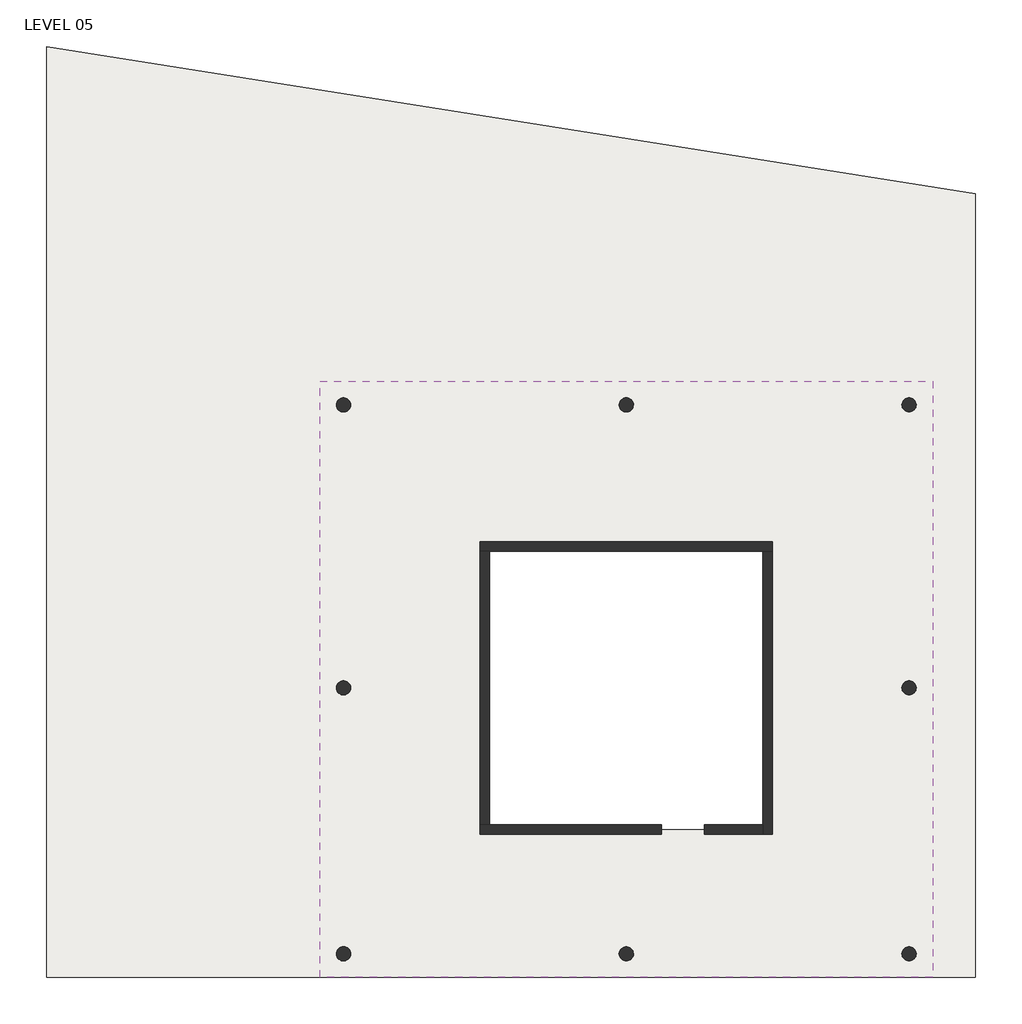
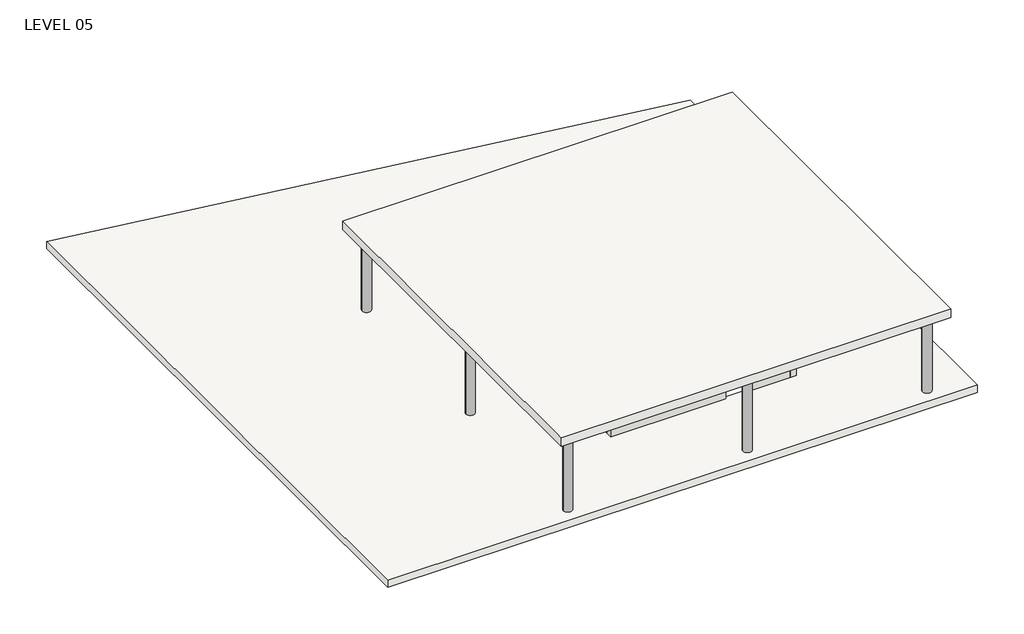
# One storey: 8 columns, 4 beams, 4 walls, 2 slabs.
"""IFC4 building model written with IfcOpenShell, lengths in millimetres."""

from ifc_helpers import new_model, si_unit, point, frame, frame_2d, origin, place, context, project, spatial, polyline, circle_curve, trimmed, segment, composite_curve, outline, extrude, faceted_brep, element, save

model = new_model("IFC4")

# Units and contexts
model_context = context("Model", 3, world=origin())
ifc_project = project(units=[si_unit("LENGTHUNIT", "METRE", prefix="MILLI")], contexts=[model_context])

# Site, building, storey
site = spatial("IfcSite", under=ifc_project)
building = spatial("IfcBuilding", under=site)
storey = spatial("IfcBuildingStorey", under=building, Name="LEVEL 05", Elevation=15000.0)

# Beams
placement = place(None, origin())
element("IfcBeam", 1, ObjectType="BHm_StructuralFraming_Concrete-RectangularBeam : 300x500 DP RC BEAM", at=placement, inside=storey, context=model_context, shape_type="SweptSolid", body=[
    extrude(outline(composite_curve([segment(polyline([(-15925.1680269, 21640.7845261), (-15925.1680269, 14640.7845261)]), True, "CONTINUOUS"), segment(trimmed(circle_curve(frame_2d((-16075.1680269, 14640.7845261)), 150.0), [point((-15925.1680269, 14640.7845261))], [point((-16225.1680269, 14640.7845261))], True, "CARTESIAN"), True, "CONTINUOUS"), segment(polyline([(-16225.1680269, 14640.7845261), (-16225.1680269, 21640.7845261)]), True, "CONTINUOUS"), segment(trimmed(circle_curve(frame_2d((-16075.1680269, 21640.7845261)), 150.0), [point((-16225.1680269, 21640.7845261))], [point((-15925.1680269, 21640.7845261))], True, "CARTESIAN"), True, "CONTINUOUS")], self_intersect=False)), frame((0.0, 0.0, 14500.0), z_axis=(0.0, 0.0, 1.0), x_axis=(1.0, 0.0, 0.0)), (0.0, 0.0, 1.0), 250.0),
])
element("IfcBeam", 2, ObjectType="BHm_StructuralFraming_Concrete-RectangularBeam : 300x500 DP RC BEAM", at=placement, inside=storey, context=model_context, shape_type="SweptSolid", body=[
    extrude(outline(composite_curve([segment(polyline([(-10925.1680269, 20840.7845261), (-10925.1680269, 14940.7845261), (-11225.1680269, 14940.7845261), (-11225.1680269, 20840.7845261)]), True, "CONTINUOUS"), segment(trimmed(circle_curve(frame_2d((-11075.1680269, 20840.7845261)), 150.0), [point((-11225.1680269, 20840.7845261))], [point((-10925.1680269, 20840.7845261))], True, "CARTESIAN"), True, "CONTINUOUS")], self_intersect=False)), frame((0.0, 0.0, 14500.0), z_axis=(0.0, 0.0, 1.0), x_axis=(1.0, 0.0, 0.0)), (0.0, 0.0, 1.0), 250.0),
])
element("IfcBeam", 3, ObjectType="BHm_StructuralFraming_Concrete-RectangularBeam : 300x500 DP RC BEAM", at=placement, inside=storey, context=model_context, shape_type="SweptSolid", body=[
    extrude(outline(composite_curve([segment(polyline([(-4925.1680269, 19840.7845261), (-4925.1680269, 14940.7845261), (-5225.1680269, 14940.7845261), (-5225.1680269, 19840.7845261)]), True, "CONTINUOUS"), segment(trimmed(circle_curve(frame_2d((-5075.1680269, 19840.7845261)), 150.0), [point((-5225.1680269, 19840.7845261))], [point((-4925.1680269, 19840.7845261))], True, "CARTESIAN"), True, "CONTINUOUS")], self_intersect=False)), frame((0.0, 0.0, 14500.0), z_axis=(0.0, 0.0, 1.0), x_axis=(1.0, 0.0, 0.0)), (0.0, 0.0, 1.0), 250.0),
])
element("IfcBeam", 4, ObjectType="BHm_StructuralFraming_Concrete-RectangularBeam : 300x500 DP RC BEAM", at=placement, inside=storey, context=model_context, shape_type="SweptSolid", body=[
    extrude(outline(composite_curve([segment(polyline([(1074.8319731, 18940.7845261), (1074.8319731, 14640.7845261)]), True, "CONTINUOUS"), segment(trimmed(circle_curve(frame_2d((924.8319731, 14640.7845261)), 150.0), [point((1074.8319731, 14640.7845261))], [point((774.8319731, 14640.7845261))], True, "CARTESIAN"), True, "CONTINUOUS"), segment(polyline([(774.8319731, 14640.7845261), (774.8319731, 18940.7845261)]), True, "CONTINUOUS"), segment(trimmed(circle_curve(frame_2d((924.8319731, 18940.7845261)), 150.0), [point((774.8319731, 18940.7845261))], [point((1074.8319731, 18940.7845261))], True, "CARTESIAN"), True, "CONTINUOUS")], self_intersect=False)), frame((0.0, 0.0, 14500.0), z_axis=(0.0, 0.0, 1.0), x_axis=(1.0, 0.0, 0.0)), (0.0, 0.0, 1.0), 250.0),
])

# Columns
element("IfcColumn", 5, ObjectType="BHm_StructuralColumns_ConcreteRound : 300 Ø RC COL", at=placement, inside=storey, context=model_context, shape_type="SweptSolid", body=[
    extrude(outline(composite_curve([segment(trimmed(circle_curve(frame_2d((-11075.1680269, 14640.7845261)), 150.0), [point((-11225.1680269, 14640.7845261))], [point((-10925.1680269, 14640.7845261))], False, "CARTESIAN"), True, "CONTINUOUS"), segment(trimmed(circle_curve(frame_2d((-11075.1680269, 14640.7845261)), 150.0), [point((-10925.1680269, 14640.7845261))], [point((-11225.1680269, 14640.7845261))], False, "CARTESIAN"), True, "CONTINUOUS")], self_intersect=False)), frame((0.0, 0.0, 15000.0), z_axis=(0.0, 0.0, 1.0), x_axis=(1.0, 0.0, 0.0)), (0.0, 0.0, 1.0), 2700.0),
])
element("IfcColumn", 6, ObjectType="BHm_StructuralColumns_ConcreteRound : 300 Ø RC COL", at=placement, inside=storey, context=model_context, shape_type="SweptSolid", body=[
    extrude(outline(composite_curve([segment(trimmed(circle_curve(frame_2d((-11075.1680269, 8640.7845261)), 150.0), [point((-11225.1680269, 8640.7845261))], [point((-10925.1680269, 8640.7845261))], False, "CARTESIAN"), True, "CONTINUOUS"), segment(trimmed(circle_curve(frame_2d((-11075.1680269, 8640.7845261)), 150.0), [point((-10925.1680269, 8640.7845261))], [point((-11225.1680269, 8640.7845261))], False, "CARTESIAN"), True, "CONTINUOUS")], self_intersect=False)), frame((0.0, 0.0, 15000.0), z_axis=(0.0, 0.0, 1.0), x_axis=(1.0, 0.0, 0.0)), (0.0, 0.0, 1.0), 2700.0),
])
element("IfcColumn", 7, ObjectType="BHm_StructuralColumns_ConcreteRound : 300 Ø RC COL", at=placement, inside=storey, context=model_context, shape_type="SweptSolid", body=[
    extrude(outline(composite_curve([segment(trimmed(circle_curve(frame_2d((-5075.1680269, 3000.0)), 150.0), [point((-5225.1680269, 3000.0))], [point((-4925.1680269, 3000.0))], False, "CARTESIAN"), True, "CONTINUOUS"), segment(trimmed(circle_curve(frame_2d((-5075.1680269, 3000.0)), 150.0), [point((-4925.1680269, 3000.0))], [point((-5225.1680269, 3000.0))], False, "CARTESIAN"), True, "CONTINUOUS")], self_intersect=False)), frame((0.0, 0.0, 15000.0), z_axis=(0.0, 0.0, 1.0), x_axis=(1.0, 0.0, 0.0)), (0.0, 0.0, 1.0), 2700.0),
])
element("IfcColumn", 8, ObjectType="BHm_StructuralColumns_ConcreteRound : 300 Ø RC COL", at=placement, inside=storey, context=model_context, shape_type="SweptSolid", body=[
    extrude(outline(composite_curve([segment(trimmed(circle_curve(frame_2d((-5075.1680269, 14640.7845261)), 150.0), [point((-5225.1680269, 14640.7845261))], [point((-4925.1680269, 14640.7845261))], False, "CARTESIAN"), True, "CONTINUOUS"), segment(trimmed(circle_curve(frame_2d((-5075.1680269, 14640.7845261)), 150.0), [point((-4925.1680269, 14640.7845261))], [point((-5225.1680269, 14640.7845261))], False, "CARTESIAN"), True, "CONTINUOUS")], self_intersect=False)), frame((0.0, 0.0, 15000.0), z_axis=(0.0, 0.0, 1.0), x_axis=(1.0, 0.0, 0.0)), (0.0, 0.0, 1.0), 2700.0),
])
element("IfcColumn", 9, ObjectType="BHm_StructuralColumns_ConcreteRound : 300 Ø RC COL", at=placement, inside=storey, context=model_context, shape_type="SweptSolid", body=[
    extrude(outline(composite_curve([segment(trimmed(circle_curve(frame_2d((924.8319731, 14640.7845261)), 150.0), [point((774.8319731, 14640.7845261))], [point((1074.8319731, 14640.7845261))], False, "CARTESIAN"), True, "CONTINUOUS"), segment(trimmed(circle_curve(frame_2d((924.8319731, 14640.7845261)), 150.0), [point((1074.8319731, 14640.7845261))], [point((774.8319731, 14640.7845261))], False, "CARTESIAN"), True, "CONTINUOUS")], self_intersect=False)), frame((0.0, 0.0, 15000.0), z_axis=(0.0, 0.0, 1.0), x_axis=(1.0, 0.0, 0.0)), (0.0, 0.0, 1.0), 2700.0),
])
element("IfcColumn", 10, ObjectType="BHm_StructuralColumns_ConcreteRound : 300 Ø RC COL", at=placement, inside=storey, context=model_context, shape_type="SweptSolid", body=[
    extrude(outline(composite_curve([segment(trimmed(circle_curve(frame_2d((924.8319731, 8640.7845261)), 150.0), [point((774.8319731, 8640.7845261))], [point((1074.8319731, 8640.7845261))], False, "CARTESIAN"), True, "CONTINUOUS"), segment(trimmed(circle_curve(frame_2d((924.8319731, 8640.7845261)), 150.0), [point((1074.8319731, 8640.7845261))], [point((774.8319731, 8640.7845261))], False, "CARTESIAN"), True, "CONTINUOUS")], self_intersect=False)), frame((0.0, 0.0, 15000.0), z_axis=(0.0, 0.0, 1.0), x_axis=(1.0, 0.0, 0.0)), (0.0, 0.0, 1.0), 2700.0),
])
element("IfcColumn", 11, ObjectType="BHm_StructuralColumns_ConcreteRound : 300 Ø RC COL", at=placement, inside=storey, context=model_context, shape_type="SweptSolid", body=[
    extrude(outline(composite_curve([segment(trimmed(circle_curve(frame_2d((924.8319731, 3000.0)), 150.0), [point((774.8319731, 3000.0))], [point((1074.8319731, 3000.0))], False, "CARTESIAN"), True, "CONTINUOUS"), segment(trimmed(circle_curve(frame_2d((924.8319731, 3000.0)), 150.0), [point((1074.8319731, 3000.0))], [point((774.8319731, 3000.0))], False, "CARTESIAN"), True, "CONTINUOUS")], self_intersect=False)), frame((0.0, 0.0, 15000.0), z_axis=(0.0, 0.0, 1.0), x_axis=(1.0, 0.0, 0.0)), (0.0, 0.0, 1.0), 2700.0),
])
element("IfcColumn", 12, ObjectType="BHm_StructuralColumns_ConcreteRound : 300 Ø RC COL", at=placement, inside=storey, context=model_context, shape_type="SweptSolid", body=[
    extrude(outline(composite_curve([segment(trimmed(circle_curve(frame_2d((-11075.1680269, 3000.0)), 150.0), [point((-11225.1680269, 3000.0))], [point((-10925.1680269, 3000.0))], False, "CARTESIAN"), True, "CONTINUOUS"), segment(trimmed(circle_curve(frame_2d((-11075.1680269, 3000.0)), 150.0), [point((-10925.1680269, 3000.0))], [point((-11225.1680269, 3000.0))], False, "CARTESIAN"), True, "CONTINUOUS")], self_intersect=False)), frame((0.0, 0.0, 15000.0), z_axis=(0.0, 0.0, 1.0), x_axis=(1.0, 0.0, 0.0)), (0.0, 0.0, 1.0), 2700.0),
])

# Slabs
element("IfcSlab", 13, ObjectType="250 THK RC SLAB", at=placement, inside=storey, context=model_context, shape_type="SweptSolid", body=[
    extrude(outline(polyline([(2324.8319731, 19120.6110517), (2324.8319731, 2500.0), (-17375.1680269, 2500.0), (-17375.1680269, 22240.7845261), (2324.8319731, 19120.6110517)]), holes=[polyline([(-2075.1680269, 11640.7845261), (-8075.1680269, 11640.7845261), (-8075.1680269, 5640.7845261), (-2075.1680269, 5640.7845261), (-2075.1680269, 11640.7845261)])]), frame((0.0, 0.0, 14750.0), z_axis=(0.0, 0.0, 1.0), x_axis=(1.0, 0.0, 0.0)), (0.0, 0.0, 1.0), 250.0),
])
element("IfcSlab", 14, ObjectType="300 THK RC SLAB", at=placement, inside=storey, context=model_context, shape_type="SweptSolid", body=[
    extrude(outline(polyline([(1424.8319731, 15140.7845261), (1424.8319731, 2500.0), (-11575.1680269, 2500.0), (-11575.1680269, 15140.7845261), (1424.8319731, 15140.7845261)])), frame((0.0, 0.0, 17700.0), z_axis=(0.0, 0.0, 1.0), x_axis=(1.0, 0.0, 0.0)), (0.0, 0.0, 1.0), 300.0),
])

# Walls
element("IfcWall", 15, ObjectType="200 THK R.C. WALL", at=placement, inside=storey, context=model_context, shape_type="Brep", body=[
    faceted_brep([(-8175.1680269, 11540.7845261, 15000.0), (-7975.1680269, 11540.7845261, 15000.0), (-2175.1680269, 11540.7845261, 15000.0), (-1975.1680269, 11540.7845261, 15000.0), (-1975.1680269, 11540.7845261, 17700.0), (-2175.1680269, 11540.7845261, 17700.0), (-7975.1680269, 11540.7845261, 17700.0), (-8175.1680269, 11540.7845261, 17700.0), (-8175.1680269, 11740.7845261, 15000.0), (-8175.1680269, 11740.7845261, 17700.0), (-1975.1680269, 11740.7845261, 17700.0), (-1975.1680269, 11740.7845261, 15000.0)], [[[0, 1, 2, 3, 4, 5, 6, 7]], [[8, 9, 10, 11]], [[3, 2, 1, 0, 8, 11]], [[4, 3, 11, 10]], [[0, 7, 9, 8]], [[7, 6, 5, 4, 10, 9]]]),
])
element("IfcWall", 16, ObjectType="200 THK R.C. WALL", at=placement, inside=storey, context=model_context, shape_type="Brep", body=[
    faceted_brep([(-2175.1680269, 11540.7845261, 15000.0), (-2175.1680269, 5740.7845261, 15000.0), (-2175.1680269, 5540.7845261, 15000.0), (-2175.1680269, 5540.7845261, 17700.0), (-2175.1680269, 5740.7845261, 17700.0), (-2175.1680269, 11540.7845261, 17700.0), (-1975.1680269, 11540.7845261, 15000.0), (-1975.1680269, 11540.7845261, 17700.0), (-1975.1680269, 5540.7845261, 17700.0), (-1975.1680269, 5540.7845261, 15000.0)], [[[0, 1, 2, 3, 4, 5]], [[6, 7, 8, 9]], [[2, 1, 0, 6, 9]], [[0, 5, 7, 6]], [[3, 2, 9, 8]], [[5, 4, 3, 8, 7]]]),
])
element("IfcWall", 17, ObjectType="200 THK R.C. WALL", at=placement, inside=storey, context=model_context, shape_type="Brep", body=[
    faceted_brep([(-2175.1680269, 5740.7845261, 15000.0), (-3417.6680269, 5740.7845261, 15000.0), (-3417.6680269, 5740.7845261, 17100.0), (-4332.6680269, 5740.7845261, 17100.0), (-4332.6680269, 5740.7845261, 15000.0), (-7975.1680269, 5740.7845261, 15000.0), (-8175.1680269, 5740.7845261, 15000.0), (-8175.1680269, 5740.7845261, 17700.0), (-7975.1680269, 5740.7845261, 17700.0), (-2175.1680269, 5740.7845261, 17700.0), (-3417.6680269, 5540.7845261, 17100.0), (-3417.6680269, 5540.7845261, 15000.0), (-2175.1680269, 5540.7845261, 15000.0), (-2175.1680269, 5540.7845261, 17700.0), (-8175.1680269, 5540.7845261, 17700.0), (-8175.1680269, 5540.7845261, 15000.0), (-4332.6680269, 5540.7845261, 15000.0), (-4332.6680269, 5540.7845261, 17100.0)], [[[0, 1, 2, 3, 4, 5, 6, 7, 8, 9]], [[10, 11, 12, 13, 14, 15, 16, 17]], [[16, 15, 6, 5, 4]], [[12, 11, 1, 0]], [[0, 9, 13, 12]], [[7, 6, 15, 14]], [[4, 3, 17, 16]], [[2, 1, 11, 10]], [[3, 2, 10, 17]], [[9, 8, 7, 14, 13]]]),
])
element("IfcWall", 18, ObjectType="200 THK R.C. WALL", at=placement, inside=storey, context=model_context, shape_type="SweptSolid", body=[
    extrude(outline(polyline([(-7975.1680269, 11540.7845261), (-7975.1680269, 5740.7845261), (-8175.1680269, 5740.7845261), (-8175.1680269, 11540.7845261), (-7975.1680269, 11540.7845261)])), frame((0.0, 0.0, 15000.0), z_axis=(0.0, 0.0, 1.0), x_axis=(1.0, 0.0, 0.0)), (0.0, 0.0, 1.0), 2700.0),
])

save(model, "model.ifc")

# Revit data of these elements
# Type "BHm_StructuralFraming_Concrete-RectangularBeam : 300x500 DP RC BEAM"
#   Keynote = "E"
#   BHE_Width = 300.000 mm
#   BHE_Length [instance default] = 1524.000 mm
#   BHE_Height = 500.000 mm
#   Length [instance default] = 1524.000 mm
#   b = 300.000 mm
#   h = 500.000 mm
#   Structural Material [instance default] = none
#   Assembly Code = ""
# Type "BHm_StructuralColumns_ConcreteRound : 300 Ø RC COL"
#   Keynote = "E"
#   b = 300.000 mm
#   BHE_Length [instance default] = 2500.000 mm
#   BHE_Diameter = 300.000 mm
#   Structural Material [instance default] = none
# Type "250 THK RC SLAB"
#   Function = 0
#   Layers, outside or top first: 250.000 mm "BHE_Concrete - Cast In-Place" (function 1)
# Type "300 THK RC SLAB"
#   Function = 0
#   Layers, outside or top first: 300.000 mm "BHE_Concrete - Cast In-Place" (function 1)
# Type "200 THK R.C. WALL"
#   Layers, outside or top first: 200.000 mm "BHE_Concrete - Cast In-Place" (function 1)
# Element 1 (IfcBeam, "BHm_StructuralFraming_Concrete-RectangularBeam : 300x500 DP RC BEAM")
#   Comments = ""
#   BHE_Length = 7000.000 mm
#   Structural Material = none
#   Phase Created = New Construction
#   Materials on its faces: "BHE_Concrete - Cast In-Place"
# Element 2 (IfcBeam, "BHm_StructuralFraming_Concrete-RectangularBeam : 300x500 DP RC BEAM")
#   Comments = ""
#   BHE_Length = 6200.000 mm
#   Structural Material = none
#   Phase Created = New Construction
#   Materials on its faces: "BHE_Concrete - Cast In-Place"
# Element 3 (IfcBeam, "BHm_StructuralFraming_Concrete-RectangularBeam : 300x500 DP RC BEAM")
#   Comments = ""
#   BHE_Length = 5200.000 mm
#   Structural Material = none
#   Phase Created = New Construction
#   Materials on its faces: "BHE_Concrete - Cast In-Place"
# Element 4 (IfcBeam, "BHm_StructuralFraming_Concrete-RectangularBeam : 300x500 DP RC BEAM")
#   Comments = ""
#   BHE_Length = 4300.000 mm
#   Structural Material = none
#   Phase Created = New Construction
#   Materials on its faces: "BHE_Concrete - Cast In-Place"
# Elements 5, 6, 7, 8, 9, 10, 11, 12 (IfcColumn, "BHm_StructuralColumns_ConcreteRound : 300 Ø RC COL")
#   Comments = ""
#   Structural Material = none
#   Phase Created = New Construction
#   Materials on its faces: "BHE_Concrete - Cast In-Place"
# Element 13 (IfcSlab, "250 THK RC SLAB")
#   Comments = ""
#   built-in parameter 1001955 = -0.15708 (stored number, unit not read)
#   Height Offset From Level = 0.000 mm
#   built-in parameter 1001954 = 1
#   Phase Created = New Construction
#   Materials on its faces: "BHE_Concrete - Cast In-Place"
# Element 14 (IfcSlab, "300 THK RC SLAB")
#   Comments = ""
#   Height Offset From Level = 3000.000 mm
#   built-in parameter 1001954 = 1
#   Phase Created = New Construction
#   Materials on its faces: "BHE_Concrete - Cast In-Place"
# Elements 15, 16, 17, 18 (IfcWall, "200 THK R.C. WALL")
#   Comments = ""
#   Top Offset = 3000.000 mm
#   Base Offset = 0.000 mm
#   wall height = 2700.000 mm
#   Phase Created = New Construction
#   Base Constraint = LEVEL 05
#   Top Constraint = LEVEL 05
#   Materials on its faces: "BHE_Concrete - Cast In-Place"
# Materials
#   "BHE_Concrete - Cast In-Place": class "Concrete", colour RGB 192 192 192, transparency 0, Cost = 0
